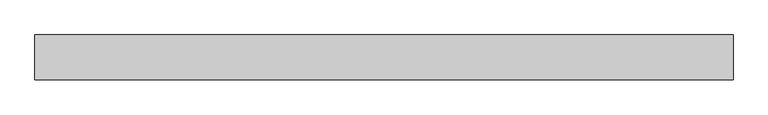
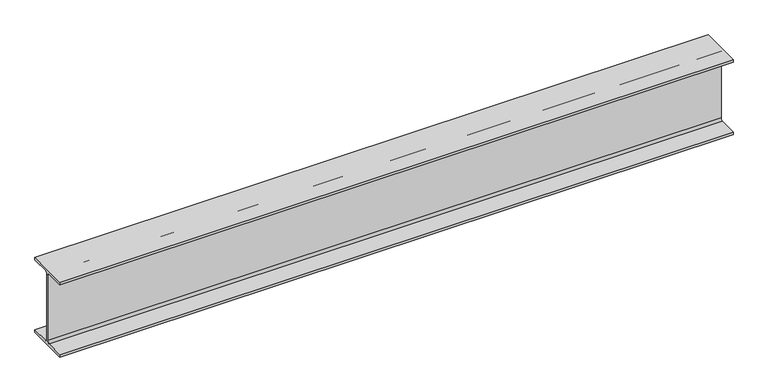
"""IFC4 building model written with IfcOpenShell, lengths in millimetres: beam geometry, Old_Steel Beam_H-KSD3502 : H_SB_ASB_H-194×150x6x9."""

from ifc_helpers import new_model, si_unit, point, frame, frame_2d, origin, place, context, project, spatial, polyline, circle_curve, trimmed, segment, composite_curve, outline, extrude, source, transform, mapped, element, save


def beam_c1192738(model_context):
    return source(origin(), model_context, "Body", "SweptSolid", [
        extrude(outline(composite_curve([segment(polyline([(82.5, -141.5), (82.5, -151.7), (-82.5, -151.7), (-82.5, -141.5), (-11.9, -141.5)]), True, "CONTINUOUS"), segment(trimmed(circle_curve(frame_2d((-11.9, -132.6)), 8.9), [point((-11.9, -141.5))], [point((-3.0, -132.6))], True, "CARTESIAN"), True, "CONTINUOUS"), segment(polyline([(-3.0, -132.6), (-3.0, 132.6)]), True, "CONTINUOUS"), segment(trimmed(circle_curve(frame_2d((-11.9, 132.6)), 8.9), [point((-3.0, 132.6))], [point((-11.9, 141.5))], True, "CARTESIAN"), True, "CONTINUOUS"), segment(polyline([(-11.9, 141.5), (-82.5, 141.5), (-82.5, 151.7), (82.5, 151.7), (82.5, 141.5), (11.9, 141.5)]), True, "CONTINUOUS"), segment(trimmed(circle_curve(frame_2d((11.9, 132.6)), 8.9), [point((11.9, 141.5))], [point((3.0, 132.6))], True, "CARTESIAN"), True, "CONTINUOUS"), segment(polyline([(3.0, 132.6), (3.0, -132.6)]), True, "CONTINUOUS"), segment(trimmed(circle_curve(frame_2d((11.9, -132.6)), 8.9), [point((3.0, -132.6))], [point((11.9, -141.5))], True, "CARTESIAN"), True, "CONTINUOUS"), segment(polyline([(11.9, -141.5), (82.5, -141.5)]), True, "CONTINUOUS")], self_intersect=False)), frame((-1265.0, 0.0, 0.0), z_axis=(1.0, 0.0, 0.0), x_axis=(0.0, 1.0, 0.0)), (0.0, 0.0, 1.0), 2578.0465428),
    ])


if __name__ == "__main__":
    model = new_model("IFC4")
    model_context = context("Model", 3, world=origin())
    ifc_project = project(units=[si_unit("LENGTHUNIT", "METRE", prefix="MILLI")], contexts=[model_context])
    site = spatial("IfcSite", under=ifc_project)
    building = spatial("IfcBuilding", under=site)
    placement = place(None, origin())
    beam_shape = beam_c1192738(model_context)
    element("IfcBeam", 1, ObjectType="Old_Steel Beam_H-KSD3502 : H_SB_ASB_H-194×150x6x9", at=placement, inside=building, context=model_context, shape_type="MappedRepresentation", body=[
        mapped(beam_shape, transform((0.0, 0.0, 0.0), x_axis=(1.0, 0.0, 0.0), y_axis=(0.0, 1.0, 0.0), z_axis=(0.0, 0.0, 1.0))),
    ])
    save(model, "model.ifc")

# Revit data of these elements
# Type "Old_Steel Beam_H-KSD3502 : H_SB_ASB_H-194×150x6x9"
#   Width = 15.0 cm
#   Web Thickness = 0.6 cm
#   Web Fillet = 1.3 cm
#   Warping Constant = 43316.0 cm⁶
#   Torsional Moment of Inertia = 8.622 cm⁴
#   Torsional Modulus = 1.0 cm³
#   Section Area = 39.01 cm²
#   Plastic Modulus weak axis = 104.0 cm³
#   Plastic Modulus strong axis = 309.0 cm³
#   Perimeter = 0.95 m²/m
#   Nominal Weight = 30.60 kgf/m
#   Moment of Inertia weak axis = 507.00 cm⁴
#   Moment of Inertia strong axis = 2690.00 cm⁴
#   Height = 19.4 cm
#   Flange Thickness = 0.9 cm
#   Elastic Modulus weak axis = 67.6 cm³
#   Elastic Modulus strong axis = 277.0 cm³
#   Centroid Vertical = 9.7 cm
#   Centroid Horizontal = 7.5 cm
#   Length [instance default] = 1.5240 m
#   Structural Material [instance default] = Steel, 45-345
#   Assembly Code = ""
# Element 1 (IfcBeam, "Old_Steel Beam_H-KSD3502 : H_SB_ASB_H-194×150x6x9")
#   Structural Material = none
# Materials
#   "Steel, 45-345": class "Metal", colour RGB 189 187 185, transparency 0, Description = "Steel 345 MPa", Cost = 0
